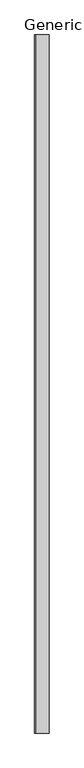
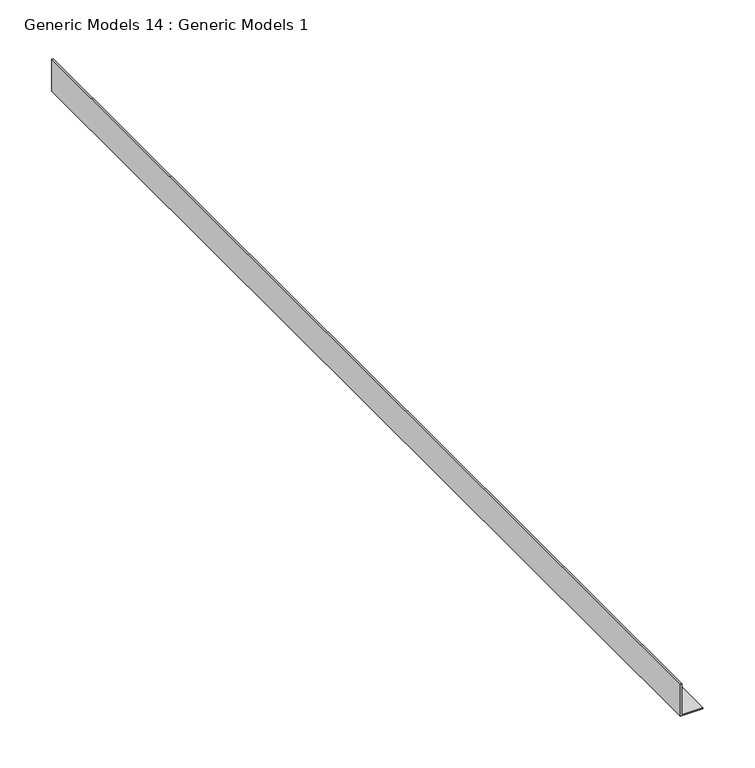
"""IFC4 building model written with IfcOpenShell, lengths in millimetres: proxy geometry, Generic Models 14 : Generic Models 1."""

import ifcopenshell
import ifcopenshell.guid

model = None  # the IFC model being written
_history = None  # IfcOwnerHistory: only IFC2X3 demands one
_inside = {}  # id of a spatial element -> (the spatial element, [elements in it])
_under = {}  # id of a project, library or spatial element -> (it, [spatial elements below it])
_declared = {}  # id of a project -> (the project, [libraries it declares])
_typed = {}  # id of a type object -> (the type object, [elements of that type])
_made_of = {}  # id of a material, layer set ... -> (it, [elements and type objects made of it])


def new_model(schema):
    """Start an empty IFC model of exactly this schema.

    Asked for "IFC4X3", IfcOpenShell would pick the latest addendum, in which some entities
    have other attributes; the version numbers below select the first issue.
    IFC2X3 requires an IfcOwnerHistory on every rooted entity: one is made here for all.
    """
    global model, _history
    if schema == "IFC4X3":
        model = ifcopenshell.file(schema_version=(4, 3, 0, 0))
    else:
        model = ifcopenshell.file(schema=schema)
    _inside.clear()
    _under.clear()
    _declared.clear()
    _typed.clear()
    _made_of.clear()
    _history = None
    if model.schema == "IFC2X3":
        org = make("IfcOrganization", Name="unknown")
        user = make(
            "IfcPersonAndOrganization",
            ThePerson=make("IfcPerson", FamilyName="unknown"),
            TheOrganization=org,
        )
        app = make(
            "IfcApplication",
            ApplicationDeveloper=org,
            Version="unknown",
            ApplicationFullName="unknown",
            ApplicationIdentifier="unknown",
        )
        _history = make(
            "IfcOwnerHistory",
            OwningUser=user,
            OwningApplication=app,
            ChangeAction="ADDED",
            CreationDate=0,
        )
    return model


def make(cls, **values):
    """One entity of the class cls with the attributes given. An attribute that is None is left unset."""
    return model.create_entity(
        cls, **{name: value for name, value in values.items() if value is not None}
    )


def rooted(cls, **values):
    """An entity with a GlobalId (a new one), such as an element, a storey or a relation."""
    return make(cls, GlobalId=ifcopenshell.guid.new(), OwnerHistory=_history, **values)


def si_unit(unit_type, name, prefix=None):
    """IfcSIUnit, for example si_unit("LENGTHUNIT", "METRE", prefix="MILLI")."""
    return make("IfcSIUnit", UnitType=unit_type, Prefix=prefix, Name=name)


def assignment(units):
    """IfcUnitAssignment: the units of a project."""
    return None if units is None else make("IfcUnitAssignment", Units=units)


def point(xyz):
    """IfcCartesianPoint."""
    return None if xyz is None else make("IfcCartesianPoint", Coordinates=xyz)


def direction(xyz):
    """IfcDirection."""
    return None if xyz is None else make("IfcDirection", DirectionRatios=xyz)


def frame(location, z_axis=None, x_axis=None):
    """IfcAxis2Placement3D, a coordinate frame: its origin and axes. An axis left out is left unset."""
    return make(
        "IfcAxis2Placement3D",
        Location=point(location),
        Axis=direction(z_axis),
        RefDirection=direction(x_axis),
    )


def origin():
    """The frame at (0, 0, 0) with its axes left unset."""
    return frame((0.0, 0.0, 0.0))


def place(relative_to, where):
    """IfcLocalPlacement: puts the frame where relative to a parent placement (None: the world)."""
    return make(
        "IfcLocalPlacement", PlacementRelTo=relative_to, RelativePlacement=where
    )


def context(
    kind, dimensions, precision=None, world=None, true_north=None, identifier=None
):
    """IfcGeometricRepresentationContext, for example the 3D "Model" context."""
    return make(
        "IfcGeometricRepresentationContext",
        ContextIdentifier=identifier,
        ContextType=kind,
        CoordinateSpaceDimension=dimensions,
        Precision=precision,
        WorldCoordinateSystem=world,
        TrueNorth=true_north,
    )


def project(units=None, contexts=None):
    """IfcProject with its units and contexts."""
    return rooted(
        "IfcProject",
        Name="project",
        RepresentationContexts=contexts,
        UnitsInContext=assignment(units),
    )


def spatial(cls, under=None, at=None, **own):
    """A site, building, storey or space (cls), placed at a placement, below another one or the project."""
    s = rooted(cls, ObjectPlacement=at, **own)
    if under is not None:
        _under.setdefault(under.id(), (under, []))[1].append(s)
    return s


def polyline(points):
    """IfcPolyline through the points."""
    return make("IfcPolyline", Points=[point(p) for p in points])


def outline(outer, holes=None, kind="AREA"):
    """IfcArbitraryClosedProfileDef: a profile drawn as a closed curve; with holes, ...WithVoids."""
    if holes is None:
        return make("IfcArbitraryClosedProfileDef", ProfileType=kind, OuterCurve=outer)
    return make(
        "IfcArbitraryProfileDefWithVoids",
        ProfileType=kind,
        OuterCurve=outer,
        InnerCurves=holes,
    )


def extrude(swept, where, along, depth):
    """IfcExtrudedAreaSolid: the profile swept, set in the frame where, extruded along a direction by depth."""
    return make(
        "IfcExtrudedAreaSolid",
        SweptArea=swept,
        Position=where,
        ExtrudedDirection=direction(along),
        Depth=depth,
    )


def shape(context_of_items, identifier, shape_type, items):
    """IfcShapeRepresentation: the items that make up one representation, for example the "Body"."""
    return make(
        "IfcShapeRepresentation",
        ContextOfItems=context_of_items,
        RepresentationIdentifier=identifier,
        RepresentationType=shape_type,
        Items=items,
    )


def source(mapping_origin, context_of_items, identifier, shape_type, items):
    """IfcRepresentationMap: a shape defined once, which mapped items show again and again."""
    return make(
        "IfcRepresentationMap",
        MappingOrigin=mapping_origin,
        MappedRepresentation=shape(context_of_items, identifier, shape_type, items),
    )


def transform(
    local_origin,
    x_axis=None,
    y_axis=None,
    z_axis=None,
    scale=None,
    scale2=None,
    scale3=None,
    uniform=True,
):
    """IfcCartesianTransformationOperator3D, or its non-uniform kind. x_axis, y_axis, z_axis: its Axis1, 2, 3."""
    if uniform:
        return make(
            "IfcCartesianTransformationOperator3D",
            Axis1=direction(x_axis),
            Axis2=direction(y_axis),
            LocalOrigin=point(local_origin),
            Scale=scale,
            Axis3=direction(z_axis),
        )
    return make(
        "IfcCartesianTransformationOperator3DnonUniform",
        Axis1=direction(x_axis),
        Axis2=direction(y_axis),
        LocalOrigin=point(local_origin),
        Scale=scale,
        Axis3=direction(z_axis),
        Scale2=scale2,
        Scale3=scale3,
    )


def mapped(mapping_source, mapping_target):
    """IfcMappedItem: shows the shape of a source again, moved by a transform."""
    return make(
        "IfcMappedItem", MappingSource=mapping_source, MappingTarget=mapping_target
    )


def made_of(thing, what):
    """Note that an element or type object is made of a material, layer set ...; save() writes the relation."""
    if what is not None:
        _made_of.setdefault(what.id(), (what, []))[1].append(thing)
    return thing


def element(
    cls,
    number,
    at=None,
    inside=None,
    cuts=None,
    type_object=None,
    material=None,
    context=None,
    identifier="Body",
    shape_type=None,
    held_by="IfcProductDefinitionShape",
    body=None,
    shapes=None,
    **own,
):
    """One element of the class cls, such as IfcWall. Its Tag is "e" and its number.

    at: its placement. inside: the storey or other place that contains it. cuts: it is an
    opening in that element (IfcRelVoidsElement). A single representation is given by context,
    identifier, shape_type and body (its items); several are given by shapes. held_by: the class
    of the entity that holds the representations. save() writes the other relations.
    """
    e = rooted(cls, Tag="e%d" % number, ObjectPlacement=at, **own)
    if body is not None:
        shapes = [shape(context, identifier, shape_type, body)]
    if shapes is not None:
        e.Representation = make(held_by, Representations=shapes)
    if inside is not None:
        _inside.setdefault(inside.id(), (inside, []))[1].append(e)
    if cuts is not None:
        rooted(
            "IfcRelVoidsElement", RelatingBuildingElement=cuts, RelatedOpeningElement=e
        )
    if type_object is not None:
        _typed.setdefault(type_object.id(), (type_object, []))[1].append(e)
    return made_of(e, material)


def aggregate(whole, parts):
    """IfcRelAggregates: a whole, such as a stair, and the parts it consists of."""
    return rooted("IfcRelAggregates", RelatingObject=whole, RelatedObjects=parts)


def save(model, path):
    """Write the relations noted so far, then the file.

    IfcRelAggregates (storeys below a building ...), IfcRelContainedInSpatialStructure (elements
    in a storey), IfcRelDefinesByType, IfcRelAssociatesMaterial and IfcRelDeclares: one each for
    every whole, place, type object, material and project.
    """
    for whole, parts in _under.values():
        aggregate(whole, parts)
    for where, things in _inside.values():
        rooted(
            "IfcRelContainedInSpatialStructure",
            RelatedElements=things,
            RelatingStructure=where,
        )
    for kind, things in _typed.values():
        rooted("IfcRelDefinesByType", RelatedObjects=things, RelatingType=kind)
    for what, things in _made_of.values():
        rooted("IfcRelAssociatesMaterial", RelatedObjects=things, RelatingMaterial=what)
    for by, libraries in _declared.values():
        rooted("IfcRelDeclares", RelatingContext=by, RelatedDefinitions=libraries)
    model.write(path)


def generic_models_14_generic_models_1_e8c90d4c(model_context):
    return source(origin(), model_context, "Body", "SweptSolid", [
        extrude(outline(polyline([(2277.1204978, 49799.875), (2239.0204978, 49799.875), (2239.0204978, 49825.275), (2240.6079978, 49825.275), (2240.6079978, 49801.4625), (2277.1204978, 49801.4625), (2277.1204978, 49799.875)])), frame((0.0, 0.0, 0.0), z_axis=(0.0, 1.0, 0.0), x_axis=(0.0, 0.0, 1.0)), (0.0, 0.0, 1.0), 1219.2),
    ])


if __name__ == "__main__":
    model = new_model("IFC4")
    model_context = context("Model", 3, world=origin())
    ifc_project = project(units=[si_unit("LENGTHUNIT", "METRE", prefix="MILLI")], contexts=[model_context])
    site = spatial("IfcSite", under=ifc_project)
    building = spatial("IfcBuilding", under=site)
    placement = place(None, origin())
    generic_models_14_generic_models_1_shape = generic_models_14_generic_models_1_e8c90d4c(model_context)
    element("IfcBuildingElementProxy", 1, Name="Generic Models 14 : Generic Models 1", ObjectType="Generic Models 14 : Generic Models 1", at=placement, inside=building, context=model_context, shape_type="MappedRepresentation", body=[
        mapped(generic_models_14_generic_models_1_shape, transform((0.0, 0.0, 0.0), x_axis=(1.0, 0.0, 0.0), y_axis=(0.0, 1.0, 0.0), z_axis=(0.0, 0.0, 1.0))),
    ])
    save(model, "model.ifc")

# Revit data of these elements
# Element 1 (IfcBuildingElementProxy, "Generic Models 14 : Generic Models 1")
#   Materials on its faces: "CEILING TRACK AS SCHEDULED"
# Materials
#   "CEILING TRACK AS SCHEDULED": class "Unassigned", colour RGB 210 209 208, transparency 0, Keynote = "M05121300.02", Cost = 0
